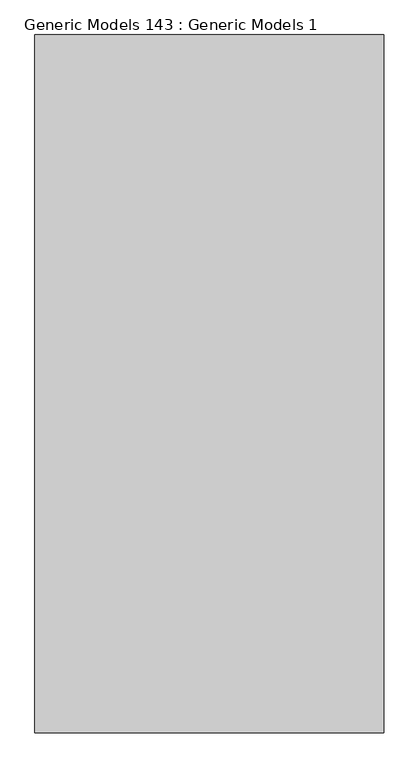
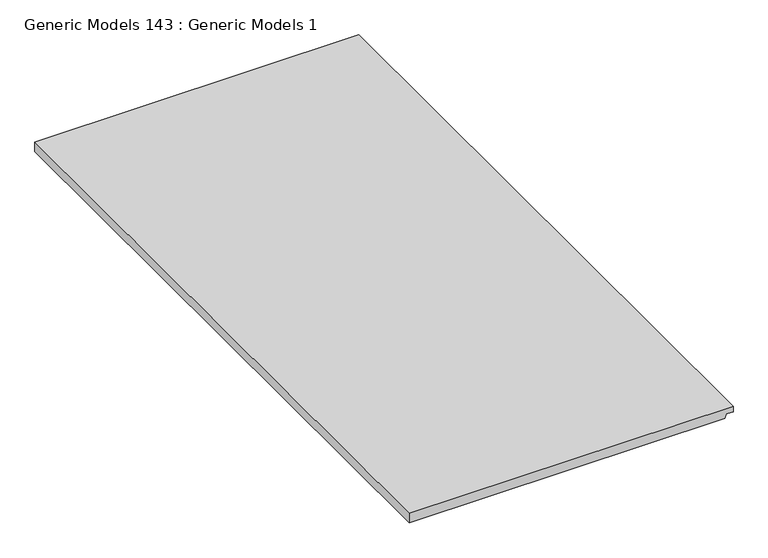
"""IFC4 building model written with IfcOpenShell, lengths in millimetres: proxy geometry, Generic Models 143 : Generic Models 1."""

from ifc_helpers import new_model, si_unit, frame, origin, place, context, project, spatial, polyline, outline, extrude, source, transform, mapped, element, save


def generic_models_143_generic_models_1_02ed30d2(model_context):
    return source(origin(), model_context, "Body", "SweptSolid", [
        extrude(outline(polyline([(2027.354361, 46814.4534123), (2027.354361, 46204.8534123), (2008.304361, 46204.8534123), (2008.304361, 46798.8643986), (2016.241861, 46801.7534123), (2016.241861, 46814.4534123), (2027.354361, 46814.4534123)])), frame((0.0, 0.0, 0.0), z_axis=(0.0, 1.0, 0.0), x_axis=(0.0, 0.0, 1.0)), (0.0, 0.0, 1.0), 1219.2),
    ])


if __name__ == "__main__":
    model = new_model("IFC4")
    model_context = context("Model", 3, world=origin())
    ifc_project = project(units=[si_unit("LENGTHUNIT", "METRE", prefix="MILLI")], contexts=[model_context])
    site = spatial("IfcSite", under=ifc_project)
    building = spatial("IfcBuilding", under=site)
    placement = place(None, origin())
    generic_models_143_generic_models_1_shape = generic_models_143_generic_models_1_02ed30d2(model_context)
    element("IfcBuildingElementProxy", 1, Name="Generic Models 143 : Generic Models 1", ObjectType="Generic Models 143 : Generic Models 1", at=placement, inside=building, context=model_context, shape_type="MappedRepresentation", body=[
        mapped(generic_models_143_generic_models_1_shape, transform((0.0, 0.0, 0.0), x_axis=(1.0, 0.0, 0.0), y_axis=(0.0, 1.0, 0.0), z_axis=(0.0, 0.0, 1.0))),
    ])
    save(model, "model.ifc")

# Revit data of these elements
# Element 1 (IfcBuildingElementProxy, "Generic Models 143 : Generic Models 1")
#   Materials on its faces: "CEILING AS SCHEDULED"
# Materials
#   "CEILING AS SCHEDULED": class "Generic", colour RGB 255 255 255, transparency 0, Cost = 0
